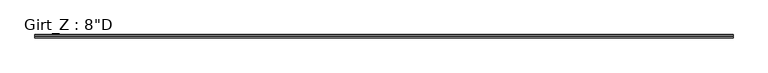
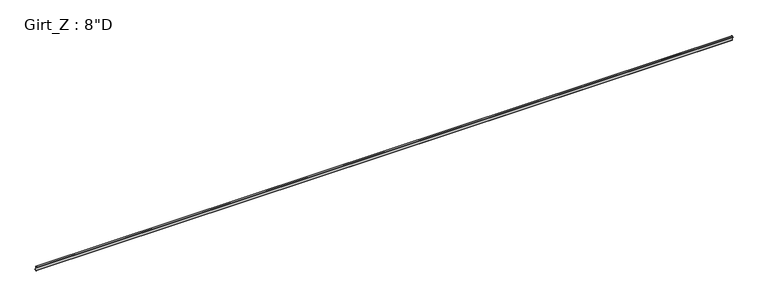
"""IFC4 building model written with IfcOpenShell, lengths in millimetres: beam geometry."""

from ifc_helpers import new_model, si_unit, point, frame, frame_2d, origin, place, context, project, spatial, polyline, circle_curve, trimmed, segment, composite_curve, outline, extrude, source, transform, mapped, element, save


def beam_ca91da87(model_context):
    return source(origin(), model_context, "Body", "SweptSolid", [
        extrude(outline(composite_curve([segment(polyline([(-63.5, 101.6), (-3.3734375, 101.6)]), True, "CONTINUOUS"), segment(trimmed(circle_curve(frame_2d((-3.3734375, 96.8375)), 4.7625), [point((-3.3734375, 101.6))], [point((1.3890625, 96.8375))], False, "CARTESIAN"), True, "CONTINUOUS"), segment(polyline([(1.3890625, 96.8375), (1.3890625, -96.8389339)]), True, "CONTINUOUS"), segment(trimmed(circle_curve(frame_2d((3.3748024, -96.8389339)), 1.9857399), [point((1.3890625, -96.8389339))], [point((3.2694106, -98.821875))], True, "CARTESIAN"), True, "CONTINUOUS"), segment(polyline([(3.2694106, -98.821875), (62.204539, -98.821875), (73.6169367, -85.221109), (75.745104, -87.0068534), (63.5, -101.6), (3.3734375, -101.6)]), True, "CONTINUOUS"), segment(trimmed(circle_curve(frame_2d((3.3734375, -96.8375)), 4.7625), [point((3.3734375, -101.6))], [point((-1.3890625, -96.8375))], False, "CARTESIAN"), True, "CONTINUOUS"), segment(polyline([(-1.3890625, -96.8375), (-1.3890625, 96.8381931)]), True, "CONTINUOUS"), segment(trimmed(circle_curve(frame_2d((-3.3741066, 96.8381931)), 1.9850441), [point((-1.3890625, 96.8381931))], [point((-3.3005807, 98.821875))], True, "CARTESIAN"), True, "CONTINUOUS"), segment(polyline([(-3.3005807, 98.821875), (-62.204539, 98.821875), (-73.6169367, 85.221109), (-75.745104, 87.0068534), (-63.5, 101.6)]), True, "CONTINUOUS")], self_intersect=False)), frame((-15624.175, 0.0, 0.0), z_axis=(1.0, 0.0, 0.0), x_axis=(0.0, 1.0, 0.0)), (0.0, 0.0, 1.0), 31235.6499994),
    ])


if __name__ == "__main__":
    model = new_model("IFC4")
    model_context = context("Model", 3, world=origin())
    ifc_project = project(units=[si_unit("LENGTHUNIT", "METRE", prefix="MILLI")], contexts=[model_context])
    site = spatial("IfcSite", under=ifc_project)
    building = spatial("IfcBuilding", under=site)
    placement = place(None, origin())
    beam_shape = beam_ca91da87(model_context)
    element("IfcBeam", 1, ObjectType="Girt_Z : 8\"D", at=placement, inside=building, context=model_context, shape_type="MappedRepresentation", body=[
        mapped(beam_shape, transform((0.0, 0.0, 0.0), x_axis=(1.0, 0.0, 0.0), y_axis=(0.0, 1.0, 0.0), z_axis=(0.0, 0.0, 1.0))),
    ])
    save(model, "model.ifc")

# Revit data of these elements
# Type "Girt_Z : 8\"D"
#   Web_Thickness = 0' - 0 7/64"
#   Length [instance default] = 10' - 0"
#   Leg_1 = 0' - 2 1/2"
#   Height = 0' - 8"
#   Structural Material [instance default] = none
# Element 1 (IfcBeam, "Girt_Z : 8\"D")
#   Structural Material = Steel
#   Materials on its faces: "Steel"
# Materials
#   "Steel": class "Metal", colour RGB 118 118 114, transparency 0, Description = "Steel, mill finish", Cost = 0
